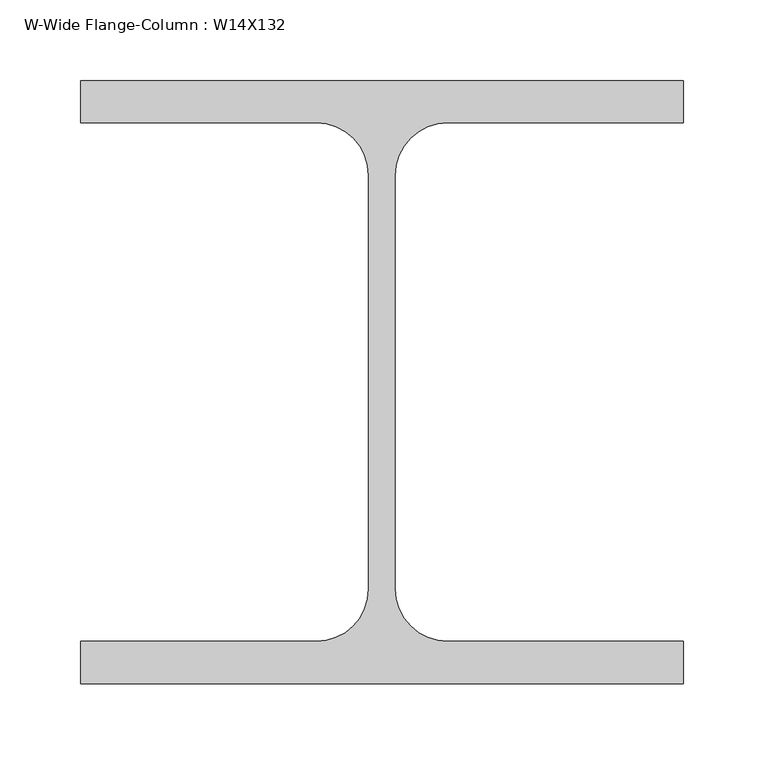
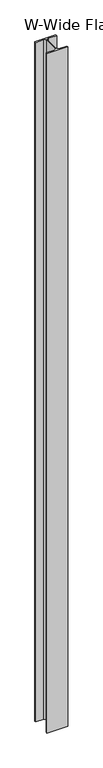
"""IFC4 building model written with IfcOpenShell, lengths in millimetres: column geometry, W-Wide Flange-Column : W14X132."""

from ifc_helpers import new_model, si_unit, point, frame, frame_2d, origin, place, context, project, spatial, polyline, circle_curve, trimmed, segment, composite_curve, outline, extrude, source, transform, mapped, element, save


def w_wide_flange_column_w14x132_ff572278(model_context):
    return source(origin(), model_context, "Body", "SweptSolid", [
        extrude(outline(composite_curve([segment(polyline([(186.69, 186.69), (186.69, 160.528), (40.767, 160.528)]), True, "CONTINUOUS"), segment(trimmed(circle_curve(frame_2d((40.767, 127.9525)), 32.5755), [point((40.767, 160.528))], [point((8.1915, 127.9525))], True, "CARTESIAN"), True, "CONTINUOUS"), segment(polyline([(8.1915, 127.9525), (8.1915, -127.9525)]), True, "CONTINUOUS"), segment(trimmed(circle_curve(frame_2d((40.767, -127.9525)), 32.5755), [point((8.1915, -127.9525))], [point((40.767, -160.528))], True, "CARTESIAN"), True, "CONTINUOUS"), segment(polyline([(40.767, -160.528), (186.69, -160.528), (186.69, -186.69), (-186.69, -186.69), (-186.69, -160.528), (-40.767, -160.528)]), True, "CONTINUOUS"), segment(trimmed(circle_curve(frame_2d((-40.767, -127.9525)), 32.5755), [point((-40.767, -160.528))], [point((-8.1915, -127.9525))], True, "CARTESIAN"), True, "CONTINUOUS"), segment(polyline([(-8.1915, -127.9525), (-8.1915, 127.9525)]), True, "CONTINUOUS"), segment(trimmed(circle_curve(frame_2d((-40.767, 127.9525)), 32.5755), [point((-8.1915, 127.9525))], [point((-40.767, 160.528))], True, "CARTESIAN"), True, "CONTINUOUS"), segment(polyline([(-40.767, 160.528), (-186.69, 160.528), (-186.69, 186.69), (186.69, 186.69)]), True, "CONTINUOUS")], self_intersect=False)), frame((0.0, 0.0, 7493.0), z_axis=(0.0, 0.0, 1.0), x_axis=(1.0, 0.0, 0.0)), (0.0, 0.0, 1.0), 12852.4),
    ])


if __name__ == "__main__":
    model = new_model("IFC4")
    model_context = context("Model", 3, world=origin())
    ifc_project = project(units=[si_unit("LENGTHUNIT", "METRE", prefix="MILLI")], contexts=[model_context])
    site = spatial("IfcSite", under=ifc_project)
    building = spatial("IfcBuilding", under=site)
    placement = place(None, origin())
    w_wide_flange_column_w14x132_shape = w_wide_flange_column_w14x132_ff572278(model_context)
    element("IfcColumn", 1, ObjectType="W-Wide Flange-Column : W14X132", at=placement, inside=building, context=model_context, shape_type="MappedRepresentation", body=[
        mapped(w_wide_flange_column_w14x132_shape, transform((0.0, 0.0, 0.0), x_axis=(1.0, 0.0, 0.0), y_axis=(0.0, 1.0, 0.0), z_axis=(0.0, 0.0, 1.0))),
    ])
    save(model, "model.ifc")

# Revit data of these elements
# Type "W-Wide Flange-Column : W14X132"
#   Assembly Code = "B10"
#   W = 132
#   bf = 1' - 2.7"
#   d = 1' - 2.7"
#   k = 0' - 2 5/16"
#   kr = 0' - 1.2825"
#   tf = 0' - 1.03"
#   tw = 0' - 0.645"
#   A = 0.269444 SF
#   Column Material [instance default] = Metal - Steel - ASTM A992
# Element 1 (IfcColumn, "W-Wide Flange-Column : W14X132")
#   Materials on its faces: "Metal - Steel - ASTM A992"
# Materials
#   "Metal - Steel - ASTM A992": class "Metal", colour RGB 128 0 0, transparency 0
